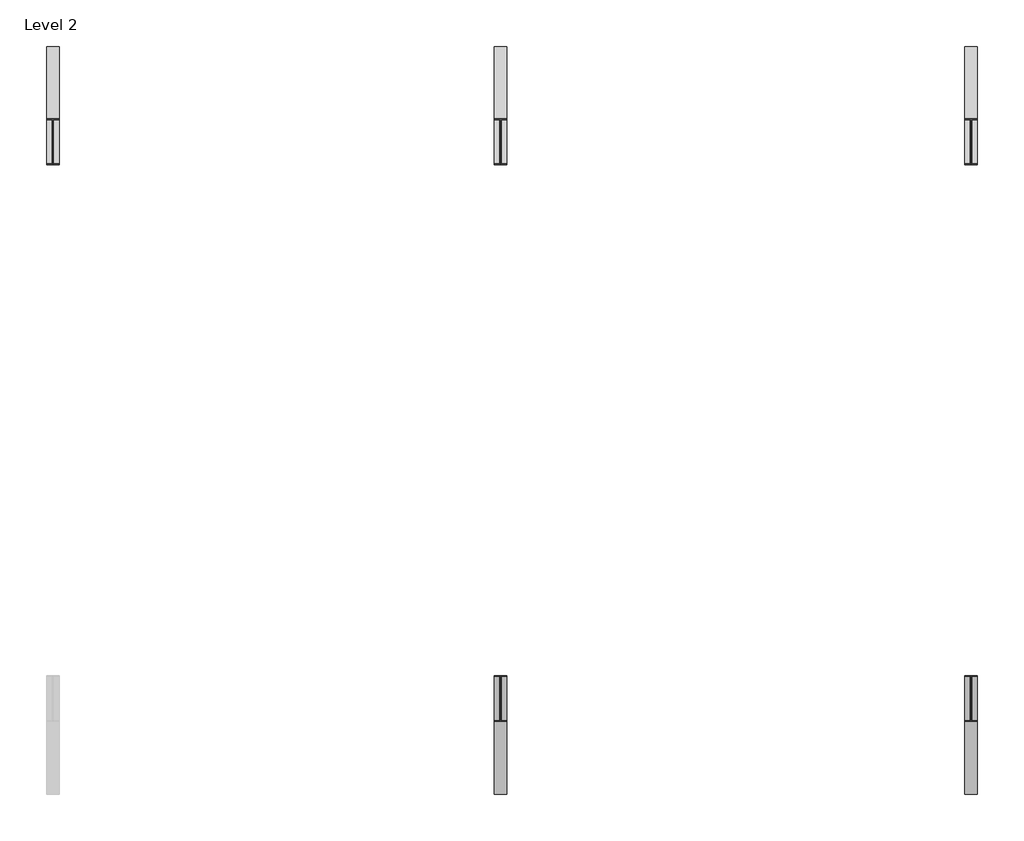
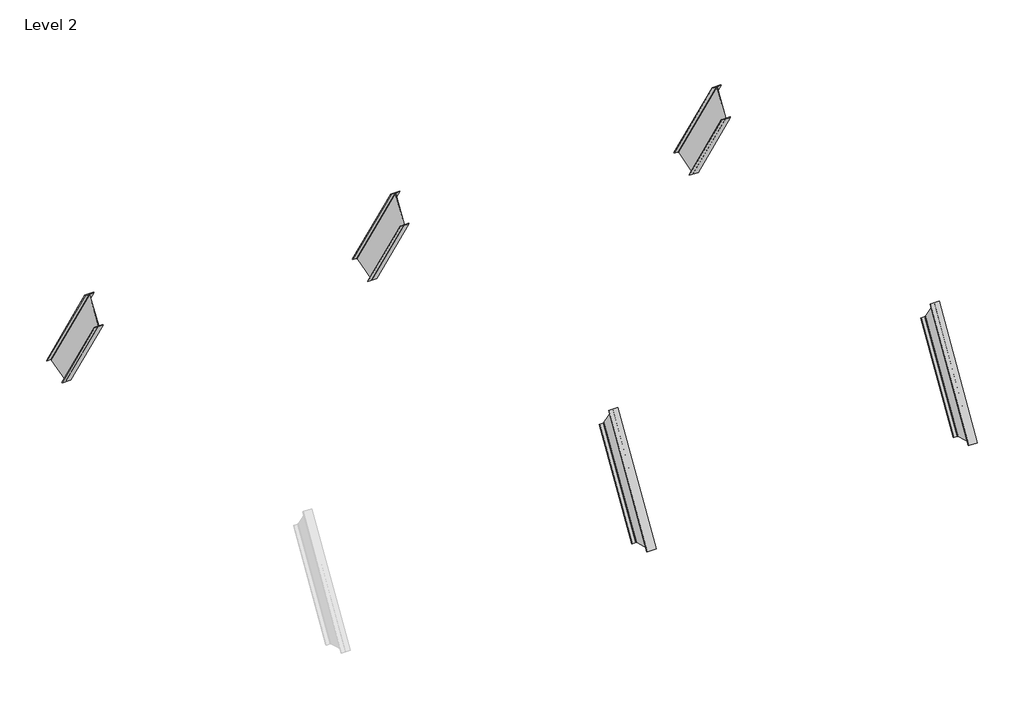
# One storey, part 2 of 2: 5 beams.
"""IFC4 building model written with IfcOpenShell, lengths in millimetres."""

from ifc_helpers import new_model, si_unit, frame, origin, place, context, project, spatial, polyline, ellipse_curve, element, save
from ifc_brep_helpers import plane_surface, revolved_surface, advanced_brep

model = new_model("IFC4")

# Units and contexts
model_context = context("Model", 3, world=origin())
ifc_project = project(units=[si_unit("LENGTHUNIT", "METRE", prefix="MILLI")], contexts=[model_context])

# Site, building, storey
site = spatial("IfcSite", under=ifc_project)
building = spatial("IfcBuilding", under=site)
storey = spatial("IfcBuildingStorey", under=building, Name="Level 2", Elevation=3048.0)

# Beams
placement = place(None, origin())
element("IfcBeam", 1, ObjectType="W Shapes : W 6X18.5", at=placement, inside=storey, context=model_context, shape_type="AdvancedBrep", body=[
    advanced_brep(
    [(28967.3280052, 10139.0601337, 4314.3781499), (29032.9870052, 10139.0601337, 4314.3781499), (29032.9870052, 11123.4136018, 2696.9143292), (28967.3280052, 11123.4136018, 2696.9143292), (28959.7080052, 10143.6843616, 4321.4371423), (28959.7080052, 11131.0336533, 2699.0506628), (28959.7080052, 10407.8819145, 4724.7409096), (28959.7080052, 11566.3925949, 2821.106522), (28967.3280052, 10412.5061424, 4731.799902), (28967.3280052, 11574.0126464, 2823.2428556), (29032.9870052, 10412.5061424, 4731.799902), (29032.9870052, 11574.0126464, 2823.2428556), (29032.9870052, 10418.3634977, 4740.7412924), (29032.9870052, 11583.6647116, 2825.9488782), (28880.5870052, 10418.3634977, 4740.7412924), (28880.5870052, 11583.6647116, 2825.9488782), (28880.5870052, 10412.5061424, 4731.799902), (28880.5870052, 11574.0126464, 2823.2428556), (28946.2460052, 10412.5061424, 4731.799902), (28946.2460052, 11574.0126464, 2823.2428556), (28953.8660052, 10407.8819145, 4724.7409096), (28953.8660052, 11566.3925949, 2821.106522), (28953.8660052, 10143.6843616, 4321.4371423), (28953.8660052, 11131.0336533, 2699.0506628), (28946.2460052, 10139.0601337, 4314.3781499), (28946.2460052, 11123.4136018, 2696.9143292), (28880.5870052, 10139.0601337, 4314.3781499), (28880.5870052, 11123.4136018, 2696.9143292), (28880.5870052, 10133.2027784, 4305.4367595), (28880.5870052, 11113.7615366, 2694.2083066), (29032.9870052, 10133.2027784, 4305.4367595), (29032.9870052, 11113.7615366, 2694.2083066)],
    [
        (0, 1),
        (1, 2),
        (2, 3),
        (3, 0),
        (4, 0, ellipse_curve(frame((28967.3280052, 10143.6843616, 4321.4371423), z_axis=(0.0, -0.836495308057375, 0.5479740866117643), x_axis=(0.0, -0.5479740866117645, -0.8364953080573748)), 8.4387711, 7.62)),
        (3, 5, ellipse_curve(frame((28967.3280052, 11131.0336533, 2699.0506628), z_axis=(0.0, 0.26994852802482067, -0.9628747541696338), x_axis=(0.0, 0.9628747541696336, 0.269948528024821)), 7.9138553, 7.62)),
        (5, 4),
        (6, 4),
        (5, 7),
        (7, 6),
        (8, 6, ellipse_curve(frame((28967.3280052, 10407.8819145, 4724.7409096), z_axis=(0.0, -0.836495308057375, 0.5479740866117643), x_axis=(0.0, -0.5479740866117645, -0.8364953080573748)), 8.4387711, 7.62)),
        (7, 9, ellipse_curve(frame((28967.3280052, 11566.3925949, 2821.106522), z_axis=(0.0, 0.26994852802482067, -0.9628747541696338), x_axis=(0.0, 0.9628747541696336, 0.269948528024821)), 7.9138553, 7.62)),
        (9, 8),
        (10, 8),
        (9, 11),
        (11, 10),
        (12, 10),
        (11, 13),
        (13, 12),
        (14, 12),
        (13, 15),
        (15, 14),
        (16, 14),
        (15, 17),
        (17, 16),
        (18, 16),
        (17, 19),
        (19, 18),
        (20, 18, ellipse_curve(frame((28946.2460052, 10407.8819145, 4724.7409096), z_axis=(0.0, -0.836495308057375, 0.5479740866117643), x_axis=(0.0, -0.5479740866117645, -0.8364953080573748)), 8.4387711, 7.62)),
        (19, 21, ellipse_curve(frame((28946.2460052, 11566.3925949, 2821.106522), z_axis=(0.0, 0.26994852802482067, -0.9628747541696338), x_axis=(0.0, 0.9628747541696336, 0.269948528024821)), 7.9138553, 7.62)),
        (21, 20),
        (22, 20),
        (21, 23),
        (23, 22),
        (24, 22, ellipse_curve(frame((28946.2460052, 10143.6843616, 4321.4371423), z_axis=(0.0, -0.836495308057375, 0.5479740866117643), x_axis=(0.0, -0.5479740866117645, -0.8364953080573748)), 8.4387711, 7.62)),
        (23, 25, ellipse_curve(frame((28946.2460052, 11131.0336533, 2699.0506628), z_axis=(0.0, 0.26994852802482067, -0.9628747541696338), x_axis=(0.0, 0.9628747541696336, 0.269948528024821)), 7.9138553, 7.62)),
        (25, 24),
        (26, 24),
        (25, 27),
        (27, 26),
        (28, 26),
        (27, 29),
        (29, 28),
        (30, 28),
        (29, 31),
        (31, 30),
        (1, 30),
        (31, 2),
    ],
    [
        plane_surface(frame((29032.9870052, 10025.1990543, 4501.4716915), z_axis=(0.0, 0.8542430559708922, 0.5198738321222864), x_axis=(0.0, 0.5198738321222864, -0.8542430559708922))),
        revolved_surface(polyline([(28959.708005200002, 11132.144372669503, 2697.225557775976), (28959.708005200002, 10141.799257339859, 4324.534696094065)]), (28967.3280052, 10031.7083863, 4505.4331301), (0.0, 0.5198738321222863, -0.8542430559708921)),
        plane_surface(frame((28959.7080052, 10031.7083863, 4505.4331301), z_axis=(1.0000000000000002, 0.0, 0.0), x_axis=(0.0, 0.5198738321222864, -0.8542430559708922))),
        revolved_surface(polyline([(28959.708005200002, 11567.50331433201, 2819.281417010493), (28959.708005200002, 10405.996810289686, 4727.8384634243885)]), (28967.3280052, 10403.6082262, 4731.7633222), (0.0, 0.5198738321222863, -0.8542430559708921)),
        plane_surface(frame((28967.3280052, 10410.1175583, 4735.7247608), z_axis=(0.0, -0.8542430559708922, -0.5198738321222864), x_axis=(0.0, 0.5198738321222864, -0.8542430559708922))),
        plane_surface(frame((29032.9870052, 10410.1175583, 4735.7247608), z_axis=(1.0000000000000002, 0.0, 0.0), x_axis=(0.0, 0.5198738321222864, -0.8542430559708922))),
        plane_surface(frame((29032.9870052, 10418.3627123, 4740.742583), z_axis=(0.0, 0.8542430559708922, 0.5198738321222864), x_axis=(0.0, 0.5198738321222864, -0.8542430559708922))),
        plane_surface(frame((28880.5870052, 10418.3627123, 4740.742583), z_axis=(-1.0000000000000002, 0.0, 0.0), x_axis=(0.0, 0.5198738321222864, -0.8542430559708922))),
        plane_surface(frame((28880.5870052, 10410.1175583, 4735.7247608), z_axis=(0.0, -0.8542430559708922, -0.5198738321222864), x_axis=(0.0, 0.5198738321222864, -0.8542430559708922))),
        revolved_surface(polyline([(28938.6260052, 11567.50331433201, 2819.281417010493), (28938.6260052, 10405.996810289686, 4727.8384634243885)]), (28946.2460052, 10403.6082262, 4731.7633222), (0.0, 0.5198738321222863, -0.8542430559708921)),
        plane_surface(frame((28953.8660052, 10403.6082262, 4731.7633222), z_axis=(-1.0000000000000002, 0.0, 0.0), x_axis=(0.0, 0.5198738321222864, -0.8542430559708922))),
        revolved_surface(polyline([(28938.6260052, 11132.144372669503, 2697.225557775976), (28938.6260052, 10141.799257339859, 4324.534696094065)]), (28946.2460052, 10031.7083863, 4505.4331301), (0.0, 0.5198738321222863, -0.8542430559708921)),
        plane_surface(frame((28946.2460052, 10025.1990543, 4501.4716915), z_axis=(0.0, 0.8542430559708922, 0.5198738321222864), x_axis=(0.0, 0.5198738321222864, -0.8542430559708922))),
        plane_surface(frame((28880.5870052, 10025.1990543, 4501.4716915), z_axis=(-1.0000000000000002, 0.0, 0.0), x_axis=(0.0, 0.5198738321222864, -0.8542430559708922))),
        plane_surface(frame((28880.5870052, 10016.9539003, 4496.4538693), z_axis=(0.0, -0.8542430559708922, -0.5198738321222864), x_axis=(0.0, 0.5198738321222864, -0.8542430559708922))),
        plane_surface(frame((29032.9870052, 10016.9539003, 4496.4538693), z_axis=(1.0000000000000002, 0.0, 0.0), x_axis=(0.0, 0.5198738321222864, -0.8542430559708922))),
        plane_surface(frame((28956.7905771, 10418.3654245, 4740.7442336), z_axis=(0.0, -0.836495308057375, 0.5479740866117643), x_axis=(1.0, 0.0, 0.0))),
        plane_surface(frame((31332.3254456, 11714.3703228, 2862.5930909), z_axis=(0.0, 0.26994852802482067, -0.9628747541696338), x_axis=(-1.0, 0.0, 0.0))),
    ],
    [
        (0, [[1, 2, 3, 4]]),
        (1, [[5, -4, 6, 7]]),
        (2, [[8, -7, 9, 10]]),
        (3, [[11, -10, 12, 13]]),
        (4, [[14, -13, 15, 16]]),
        (5, [[17, -16, 18, 19]]),
        (6, [[20, -19, 21, 22]]),
        (7, [[23, -22, 24, 25]]),
        (8, [[26, -25, 27, 28]]),
        (9, [[29, -28, 30, 31]]),
        (10, [[32, -31, 33, 34]]),
        (11, [[35, -34, 36, 37]]),
        (12, [[38, -37, 39, 40]]),
        (13, [[41, -40, 42, 43]]),
        (14, [[44, -43, 45, 46]]),
        (15, [[47, -46, 48, -2]]),
        (16, [[-1, -5, -8, -11, -14, -17, -20, -23, -26, -29, -32, -35, -38, -41, -44, -47]]),
        (17, [[-3, -48, -45, -42, -39, -36, -33, -30, -27, -24, -21, -18, -15, -12, -9, -6]]),
    ],
),
])
element("IfcBeam", 2, ObjectType="W Shapes : W 6X18.5", at=placement, inside=storey, context=model_context, shape_type="AdvancedBrep", body=[
    advanced_brep(
    [(29032.9870052, 4087.4629396, 4314.3781499), (28967.3280052, 4087.4629396, 4314.3781499), (28967.3280052, 3103.1094714, 2696.9143292), (29032.9870052, 3103.1094714, 2696.9143292), (28959.7080052, 4082.8387117, 4321.4371423), (28959.7080052, 3095.4894199, 2699.0506628), (28959.7080052, 3818.6411587, 4724.7409096), (28959.7080052, 2660.1304783, 2821.106522), (28967.3280052, 3814.0169308, 4731.799902), (28967.3280052, 2652.5104268, 2823.2428556), (29032.9870052, 3814.0169308, 4731.799902), (29032.9870052, 2652.5104268, 2823.2428556), (29032.9870052, 3808.1595755, 4740.7412924), (29032.9870052, 2642.8583616, 2825.9488782), (28880.5870052, 3808.1595755, 4740.7412924), (28880.5870052, 2642.8583616, 2825.9488782), (28880.5870052, 3814.0169308, 4731.799902), (28880.5870052, 2652.5104268, 2823.2428556), (28946.2460052, 3814.0169308, 4731.799902), (28946.2460052, 2652.5104268, 2823.2428556), (28953.8660052, 3818.6411587, 4724.7409096), (28953.8660052, 2660.1304783, 2821.106522), (28953.8660052, 4082.8387117, 4321.4371423), (28953.8660052, 3095.4894199, 2699.0506628), (28946.2460052, 4087.4629396, 4314.3781499), (28946.2460052, 3103.1094714, 2696.9143292), (28880.5870052, 4087.4629396, 4314.3781499), (28880.5870052, 3103.1094714, 2696.9143292), (28880.5870052, 4093.3202949, 4305.4367595), (28880.5870052, 3112.7615366, 2694.2083066), (29032.9870052, 4093.3202949, 4305.4367595), (29032.9870052, 3112.7615366, 2694.2083066)],
    [
        (0, 1),
        (1, 2),
        (2, 3),
        (3, 0),
        (1, 4, ellipse_curve(frame((28967.3280052, 4082.8387117, 4321.4371423), z_axis=(0.0, 0.8364953080573764, 0.5479740866117624), x_axis=(0.0, 0.5479740866117631, -0.8364953080573758)), 8.4387711, 7.62)),
        (4, 5),
        (5, 2, ellipse_curve(frame((28967.3280052, 3095.4894199, 2699.0506628), z_axis=(0.0, -0.26994852802482067, -0.9628747541696338), x_axis=(0.0, -0.9628747541696336, 0.26994852802482094)), 7.9138553, 7.62)),
        (4, 6),
        (6, 7),
        (7, 5),
        (6, 8, ellipse_curve(frame((28967.3280052, 3818.6411587, 4724.7409096), z_axis=(0.0, 0.8364953080573764, 0.5479740866117624), x_axis=(0.0, 0.5479740866117631, -0.8364953080573758)), 8.4387711, 7.62)),
        (8, 9),
        (9, 7, ellipse_curve(frame((28967.3280052, 2660.1304783, 2821.106522), z_axis=(0.0, -0.26994852802482067, -0.9628747541696338), x_axis=(0.0, -0.9628747541696336, 0.26994852802482094)), 7.9138553, 7.62)),
        (8, 10),
        (10, 11),
        (11, 9),
        (10, 12),
        (12, 13),
        (13, 11),
        (12, 14),
        (14, 15),
        (15, 13),
        (14, 16),
        (16, 17),
        (17, 15),
        (16, 18),
        (18, 19),
        (19, 17),
        (18, 20, ellipse_curve(frame((28946.2460052, 3818.6411587, 4724.7409096), z_axis=(0.0, 0.8364953080573764, 0.5479740866117624), x_axis=(0.0, 0.5479740866117631, -0.8364953080573758)), 8.4387711, 7.62)),
        (20, 21),
        (21, 19, ellipse_curve(frame((28946.2460052, 2660.1304783, 2821.106522), z_axis=(0.0, -0.26994852802482067, -0.9628747541696338), x_axis=(0.0, -0.9628747541696336, 0.26994852802482094)), 7.9138553, 7.62)),
        (20, 22),
        (22, 23),
        (23, 21),
        (22, 24, ellipse_curve(frame((28946.2460052, 4082.8387117, 4321.4371423), z_axis=(0.0, 0.8364953080573764, 0.5479740866117624), x_axis=(0.0, 0.5479740866117631, -0.8364953080573758)), 8.4387711, 7.62)),
        (24, 25),
        (25, 23, ellipse_curve(frame((28946.2460052, 3095.4894199, 2699.0506628), z_axis=(0.0, -0.26994852802482067, -0.9628747541696338), x_axis=(0.0, -0.9628747541696336, 0.26994852802482094)), 7.9138553, 7.62)),
        (24, 26),
        (26, 27),
        (27, 25),
        (26, 28),
        (28, 29),
        (29, 27),
        (28, 30),
        (30, 31),
        (31, 29),
        (30, 0),
        (3, 31),
    ],
    [
        plane_surface(frame((29032.9870052, 4201.324019, 4501.4716915), z_axis=(0.0, -0.8542430559708922, 0.5198738321222864), x_axis=(0.0, -0.5198738321222864, -0.8542430559708922))),
        revolved_surface(polyline([(28959.708005200002, 3094.3787005304976, 2697.225557775975), (28959.708005200002, 4084.7238158871687, 4324.534696138475)]), (28967.3280052, 4194.8146869, 4505.4331301), (0.0, -0.5198738321222864, -0.8542430559708922)),
        plane_surface(frame((28959.7080052, 4194.8146869, 4505.4331301), z_axis=(1.0000000000000002, 0.0, 0.0), x_axis=(0.0, -0.5198738321222864, -0.8542430559708922))),
        revolved_surface(polyline([(28959.708005200002, 2659.0197588679885, 2819.2814170104925), (28959.708005200002, 3820.5262629103145, 4727.8384634243885)]), (28967.3280052, 3822.914847, 4731.7633222), (0.0, -0.5198738321222864, -0.8542430559708922)),
        plane_surface(frame((28967.3280052, 3816.405515, 4735.7247608), z_axis=(0.0, 0.8542430559708922, -0.5198738321222864), x_axis=(0.0, -0.5198738321222864, -0.8542430559708922))),
        plane_surface(frame((29032.9870052, 3816.405515, 4735.7247608), z_axis=(1.0000000000000002, 0.0, 0.0), x_axis=(0.0, -0.5198738321222864, -0.8542430559708922))),
        plane_surface(frame((29032.9870052, 3808.160361, 4740.742583), z_axis=(0.0, -0.8542430559708922, 0.5198738321222864), x_axis=(0.0, -0.5198738321222864, -0.8542430559708922))),
        plane_surface(frame((28880.5870052, 3808.160361, 4740.742583), z_axis=(-1.0000000000000002, 0.0, 0.0), x_axis=(0.0, -0.5198738321222864, -0.8542430559708922))),
        plane_surface(frame((28880.5870052, 3816.405515, 4735.7247608), z_axis=(0.0, 0.8542430559708922, -0.5198738321222864), x_axis=(0.0, -0.5198738321222864, -0.8542430559708922))),
        revolved_surface(polyline([(28938.6260052, 2659.0197588679885, 2819.2814170104925), (28938.6260052, 3820.5262629103145, 4727.8384634243885)]), (28946.2460052, 3822.914847, 4731.7633222), (0.0, -0.5198738321222864, -0.8542430559708922)),
        plane_surface(frame((28953.8660052, 3822.914847, 4731.7633222), z_axis=(-1.0000000000000002, 0.0, 0.0), x_axis=(0.0, -0.5198738321222864, -0.8542430559708922))),
        revolved_surface(polyline([(28938.6260052, 3094.3787005304976, 2697.225557775975), (28938.6260052, 4084.7238158871687, 4324.534696138475)]), (28946.2460052, 4194.8146869, 4505.4331301), (0.0, -0.5198738321222864, -0.8542430559708922)),
        plane_surface(frame((28946.2460052, 4201.324019, 4501.4716915), z_axis=(0.0, -0.8542430559708922, 0.5198738321222864), x_axis=(0.0, -0.5198738321222864, -0.8542430559708922))),
        plane_surface(frame((28880.5870052, 4201.324019, 4501.4716915), z_axis=(-1.0000000000000002, 0.0, 0.0), x_axis=(0.0, -0.5198738321222864, -0.8542430559708922))),
        plane_surface(frame((28880.5870052, 4209.569173, 4496.4538693), z_axis=(0.0, 0.8542430559708922, -0.5198738321222864), x_axis=(0.0, -0.5198738321222864, -0.8542430559708922))),
        plane_surface(frame((29032.9870052, 4209.569173, 4496.4538693), z_axis=(1.0000000000000002, 0.0, 0.0), x_axis=(0.0, -0.5198738321222864, -0.8542430559708922))),
        plane_surface(frame((26581.2485648, 2512.1527504, 2862.5930909), z_axis=(0.0, -0.26994852802482067, -0.9628747541696338), x_axis=(1.0, 0.0, 0.0))),
        plane_surface(frame((28956.7905771, 4093.3183681, 4305.4397008), z_axis=(0.0, 0.8364953080573764, 0.5479740866117624), x_axis=(1.0, 0.0, 0.0))),
    ],
    [
        (0, [[1, 2, 3, 4]]),
        (1, [[5, 6, 7, -2]]),
        (2, [[8, 9, 10, -6]]),
        (3, [[11, 12, 13, -9]]),
        (4, [[14, 15, 16, -12]]),
        (5, [[17, 18, 19, -15]]),
        (6, [[20, 21, 22, -18]]),
        (7, [[23, 24, 25, -21]]),
        (8, [[26, 27, 28, -24]]),
        (9, [[29, 30, 31, -27]]),
        (10, [[32, 33, 34, -30]]),
        (11, [[35, 36, 37, -33]]),
        (12, [[38, 39, 40, -36]]),
        (13, [[41, 42, 43, -39]]),
        (14, [[44, 45, 46, -42]]),
        (15, [[47, -4, 48, -45]]),
        (16, [[-3, -7, -10, -13, -16, -19, -22, -25, -28, -31, -34, -37, -40, -43, -46, -48]]),
        (17, [[-1, -47, -44, -41, -38, -35, -32, -29, -26, -23, -20, -17, -14, -11, -8, -5]]),
    ],
),
])
element("IfcBeam", 3, ObjectType="W Shapes : W 6X18.5", at=placement, inside=storey, context=model_context, shape_type="AdvancedBrep", body=[
    advanced_brep(
    [(23341.2280052, 10139.0601337, 4314.3781499), (23406.8870052, 10139.0601337, 4314.3781499), (23406.8870052, 11123.4136018, 2696.9143292), (23341.2280052, 11123.4136018, 2696.9143292), (23333.6080052, 10143.6843616, 4321.4371423), (23333.6080052, 11131.0336533, 2699.0506628), (23333.6080052, 10407.8819145, 4724.7409096), (23333.6080052, 11566.3925949, 2821.106522), (23341.2280052, 10412.5061424, 4731.799902), (23341.2280052, 11574.0126464, 2823.2428556), (23406.8870052, 10412.5061424, 4731.799902), (23406.8870052, 11574.0126464, 2823.2428556), (23406.8870052, 10418.3634977, 4740.7412924), (23406.8870052, 11583.6647116, 2825.9488782), (23254.4870052, 10418.3634977, 4740.7412924), (23254.4870052, 11583.6647116, 2825.9488782), (23254.4870052, 10412.5061424, 4731.799902), (23254.4870052, 11574.0126464, 2823.2428556), (23320.1460052, 10412.5061424, 4731.799902), (23320.1460052, 11574.0126464, 2823.2428556), (23327.7660052, 10407.8819145, 4724.7409096), (23327.7660052, 11566.3925949, 2821.106522), (23327.7660052, 10143.6843616, 4321.4371423), (23327.7660052, 11131.0336533, 2699.0506628), (23320.1460052, 10139.0601337, 4314.3781499), (23320.1460052, 11123.4136018, 2696.9143292), (23254.4870052, 10139.0601337, 4314.3781499), (23254.4870052, 11123.4136018, 2696.9143292), (23254.4870052, 10133.2027784, 4305.4367595), (23254.4870052, 11113.7615366, 2694.2083066), (23406.8870052, 10133.2027784, 4305.4367595), (23406.8870052, 11113.7615366, 2694.2083066)],
    [
        (0, 1),
        (1, 2),
        (2, 3),
        (3, 0),
        (4, 0, ellipse_curve(frame((23341.2280052, 10143.6843616, 4321.4371423), z_axis=(0.0, -0.836495308057375, 0.5479740866117643), x_axis=(0.0, -0.5479740866117645, -0.8364953080573748)), 8.4387711, 7.62)),
        (3, 5, ellipse_curve(frame((23341.2280052, 11131.0336533, 2699.0506628), z_axis=(0.0, 0.2699485280248213, -0.9628747541696336), x_axis=(0.0, 0.9628747541696333, 0.26994852802482194)), 7.9138553, 7.62)),
        (5, 4),
        (6, 4),
        (5, 7),
        (7, 6),
        (8, 6, ellipse_curve(frame((23341.2280052, 10407.8819145, 4724.7409096), z_axis=(0.0, -0.836495308057375, 0.5479740866117643), x_axis=(0.0, -0.5479740866117645, -0.8364953080573748)), 8.4387711, 7.62)),
        (7, 9, ellipse_curve(frame((23341.2280052, 11566.3925949, 2821.106522), z_axis=(0.0, 0.2699485280248213, -0.9628747541696336), x_axis=(0.0, 0.9628747541696333, 0.26994852802482194)), 7.9138553, 7.62)),
        (9, 8),
        (10, 8),
        (9, 11),
        (11, 10),
        (12, 10),
        (11, 13),
        (13, 12),
        (14, 12),
        (13, 15),
        (15, 14),
        (16, 14),
        (15, 17),
        (17, 16),
        (18, 16),
        (17, 19),
        (19, 18),
        (20, 18, ellipse_curve(frame((23320.1460052, 10407.8819145, 4724.7409096), z_axis=(0.0, -0.836495308057375, 0.5479740866117643), x_axis=(0.0, -0.5479740866117645, -0.8364953080573748)), 8.4387711, 7.62)),
        (19, 21, ellipse_curve(frame((23320.1460052, 11566.3925949, 2821.106522), z_axis=(0.0, 0.2699485280248213, -0.9628747541696336), x_axis=(0.0, 0.9628747541696333, 0.26994852802482194)), 7.9138553, 7.62)),
        (21, 20),
        (22, 20),
        (21, 23),
        (23, 22),
        (24, 22, ellipse_curve(frame((23320.1460052, 10143.6843616, 4321.4371423), z_axis=(0.0, -0.836495308057375, 0.5479740866117643), x_axis=(0.0, -0.5479740866117645, -0.8364953080573748)), 8.4387711, 7.62)),
        (23, 25, ellipse_curve(frame((23320.1460052, 11131.0336533, 2699.0506628), z_axis=(0.0, 0.2699485280248213, -0.9628747541696336), x_axis=(0.0, 0.9628747541696333, 0.26994852802482194)), 7.9138553, 7.62)),
        (25, 24),
        (26, 24),
        (25, 27),
        (27, 26),
        (28, 26),
        (27, 29),
        (29, 28),
        (30, 28),
        (29, 31),
        (31, 30),
        (1, 30),
        (31, 2),
    ],
    [
        plane_surface(frame((23406.8870052, 10025.1990543, 4501.4716915), z_axis=(0.0, 0.8542430559708922, 0.5198738321222864), x_axis=(0.0, 0.5198738321222864, -0.8542430559708922))),
        revolved_surface(polyline([(23333.6080052, 11132.144372669503, 2697.225557775976), (23333.6080052, 10141.799257339859, 4324.534696094065)]), (23341.2280052, 10031.7083863, 4505.4331301), (0.0, 0.5198738321222863, -0.8542430559708921)),
        plane_surface(frame((23333.6080052, 10031.7083863, 4505.4331301), z_axis=(1.0000000000000002, 0.0, 0.0), x_axis=(0.0, 0.5198738321222864, -0.8542430559708922))),
        revolved_surface(polyline([(23333.6080052, 11567.50331433201, 2819.281417010493), (23333.6080052, 10405.996810289686, 4727.8384634243885)]), (23341.2280052, 10403.6082262, 4731.7633222), (0.0, 0.5198738321222863, -0.8542430559708921)),
        plane_surface(frame((23341.2280052, 10410.1175583, 4735.7247608), z_axis=(0.0, -0.8542430559708922, -0.5198738321222864), x_axis=(0.0, 0.5198738321222864, -0.8542430559708922))),
        plane_surface(frame((23406.8870052, 10410.1175583, 4735.7247608), z_axis=(1.0000000000000002, 0.0, 0.0), x_axis=(0.0, 0.5198738321222864, -0.8542430559708922))),
        plane_surface(frame((23406.8870052, 10418.3627123, 4740.742583), z_axis=(0.0, 0.8542430559708922, 0.5198738321222864), x_axis=(0.0, 0.5198738321222864, -0.8542430559708922))),
        plane_surface(frame((23254.4870052, 10418.3627123, 4740.742583), z_axis=(-1.0000000000000002, 0.0, 0.0), x_axis=(0.0, 0.5198738321222864, -0.8542430559708922))),
        plane_surface(frame((23254.4870052, 10410.1175583, 4735.7247608), z_axis=(0.0, -0.8542430559708922, -0.5198738321222864), x_axis=(0.0, 0.5198738321222864, -0.8542430559708922))),
        revolved_surface(polyline([(23312.5260052, 11567.50331433201, 2819.281417010493), (23312.5260052, 10405.996810289686, 4727.8384634243885)]), (23320.1460052, 10403.6082262, 4731.7633222), (0.0, 0.5198738321222863, -0.8542430559708921)),
        plane_surface(frame((23327.7660052, 10403.6082262, 4731.7633222), z_axis=(-1.0000000000000002, 0.0, 0.0), x_axis=(0.0, 0.5198738321222864, -0.8542430559708922))),
        revolved_surface(polyline([(23312.5260052, 11132.144372669503, 2697.225557775976), (23312.5260052, 10141.799257339859, 4324.534696094065)]), (23320.1460052, 10031.7083863, 4505.4331301), (0.0, 0.5198738321222863, -0.8542430559708921)),
        plane_surface(frame((23320.1460052, 10025.1990543, 4501.4716915), z_axis=(0.0, 0.8542430559708922, 0.5198738321222864), x_axis=(0.0, 0.5198738321222864, -0.8542430559708922))),
        plane_surface(frame((23254.4870052, 10025.1990543, 4501.4716915), z_axis=(-1.0000000000000002, 0.0, 0.0), x_axis=(0.0, 0.5198738321222864, -0.8542430559708922))),
        plane_surface(frame((23254.4870052, 10016.9539003, 4496.4538693), z_axis=(0.0, -0.8542430559708922, -0.5198738321222864), x_axis=(0.0, 0.5198738321222864, -0.8542430559708922))),
        plane_surface(frame((23406.8870052, 10016.9539003, 4496.4538693), z_axis=(1.0000000000000002, 0.0, 0.0), x_axis=(0.0, 0.5198738321222864, -0.8542430559708922))),
        plane_surface(frame((25706.2254456, 11714.3703228, 2862.5930909), z_axis=(0.0, 0.2699485280248213, -0.9628747541696336), x_axis=(-1.0, 0.0, 0.0))),
        plane_surface(frame((23330.6905771, 10418.3654245, 4740.7442336), z_axis=(0.0, -0.836495308057375, 0.5479740866117643), x_axis=(1.0, 0.0, 0.0))),
    ],
    [
        (0, [[1, 2, 3, 4]]),
        (1, [[5, -4, 6, 7]]),
        (2, [[8, -7, 9, 10]]),
        (3, [[11, -10, 12, 13]]),
        (4, [[14, -13, 15, 16]]),
        (5, [[17, -16, 18, 19]]),
        (6, [[20, -19, 21, 22]]),
        (7, [[23, -22, 24, 25]]),
        (8, [[26, -25, 27, 28]]),
        (9, [[29, -28, 30, 31]]),
        (10, [[32, -31, 33, 34]]),
        (11, [[35, -34, 36, 37]]),
        (12, [[38, -37, 39, 40]]),
        (13, [[41, -40, 42, 43]]),
        (14, [[44, -43, 45, 46]]),
        (15, [[47, -46, 48, -2]]),
        (16, [[-3, -48, -45, -42, -39, -36, -33, -30, -27, -24, -21, -18, -15, -12, -9, -6]]),
        (17, [[-1, -5, -8, -11, -14, -17, -20, -23, -26, -29, -32, -35, -38, -41, -44, -47]]),
    ],
),
])
element("IfcBeam", 4, ObjectType="W Shapes : W 6X18.5", at=placement, inside=storey, context=model_context, shape_type="AdvancedBrep", body=[
    advanced_brep(
    [(23406.8870052, 4087.4629396, 4314.3781499), (23341.2280052, 4087.4629396, 4314.3781499), (23341.2280052, 3103.1094714, 2696.9143292), (23406.8870052, 3103.1094714, 2696.9143292), (23333.6080052, 4082.8387117, 4321.4371423), (23333.6080052, 3095.4894199, 2699.0506628), (23333.6080052, 3818.6411587, 4724.7409096), (23333.6080052, 2660.1304783, 2821.106522), (23341.2280052, 3814.0169308, 4731.799902), (23341.2280052, 2652.5104268, 2823.2428556), (23406.8870052, 3814.0169308, 4731.799902), (23406.8870052, 2652.5104268, 2823.2428556), (23406.8870052, 3808.1595755, 4740.7412924), (23406.8870052, 2642.8583616, 2825.9488782), (23254.4870052, 3808.1595755, 4740.7412924), (23254.4870052, 2642.8583616, 2825.9488782), (23254.4870052, 3814.0169308, 4731.799902), (23254.4870052, 2652.5104268, 2823.2428556), (23320.1460052, 3814.0169308, 4731.799902), (23320.1460052, 2652.5104268, 2823.2428556), (23327.7660052, 3818.6411587, 4724.7409096), (23327.7660052, 2660.1304783, 2821.106522), (23327.7660052, 4082.8387117, 4321.4371423), (23327.7660052, 3095.4894199, 2699.0506628), (23320.1460052, 4087.4629396, 4314.3781499), (23320.1460052, 3103.1094714, 2696.9143292), (23254.4870052, 4087.4629396, 4314.3781499), (23254.4870052, 3103.1094714, 2696.9143292), (23254.4870052, 4093.3202949, 4305.4367595), (23254.4870052, 3112.7615366, 2694.2083066), (23406.8870052, 4093.3202949, 4305.4367595), (23406.8870052, 3112.7615366, 2694.2083066)],
    [
        (0, 1),
        (1, 2),
        (2, 3),
        (3, 0),
        (1, 4, ellipse_curve(frame((23341.2280052, 4082.8387117, 4321.4371423), z_axis=(0.0, 0.8364953080573764, 0.5479740866117624), x_axis=(0.0, 0.5479740866117631, -0.8364953080573758)), 8.4387711, 7.62)),
        (4, 5),
        (5, 2, ellipse_curve(frame((23341.2280052, 3095.4894199, 2699.0506628), z_axis=(0.0, -0.26994852802482067, -0.9628747541696338), x_axis=(0.0, -0.9628747541696336, 0.26994852802482094)), 7.9138553, 7.62)),
        (4, 6),
        (6, 7),
        (7, 5),
        (6, 8, ellipse_curve(frame((23341.2280052, 3818.6411587, 4724.7409096), z_axis=(0.0, 0.8364953080573764, 0.5479740866117624), x_axis=(0.0, 0.5479740866117631, -0.8364953080573758)), 8.4387711, 7.62)),
        (8, 9),
        (9, 7, ellipse_curve(frame((23341.2280052, 2660.1304783, 2821.106522), z_axis=(0.0, -0.26994852802482067, -0.9628747541696338), x_axis=(0.0, -0.9628747541696336, 0.26994852802482094)), 7.9138553, 7.62)),
        (8, 10),
        (10, 11),
        (11, 9),
        (10, 12),
        (12, 13),
        (13, 11),
        (12, 14),
        (14, 15),
        (15, 13),
        (14, 16),
        (16, 17),
        (17, 15),
        (16, 18),
        (18, 19),
        (19, 17),
        (18, 20, ellipse_curve(frame((23320.1460052, 3818.6411587, 4724.7409096), z_axis=(0.0, 0.8364953080573764, 0.5479740866117624), x_axis=(0.0, 0.5479740866117631, -0.8364953080573758)), 8.4387711, 7.62)),
        (20, 21),
        (21, 19, ellipse_curve(frame((23320.1460052, 2660.1304783, 2821.106522), z_axis=(0.0, -0.26994852802482067, -0.9628747541696338), x_axis=(0.0, -0.9628747541696336, 0.26994852802482094)), 7.9138553, 7.62)),
        (20, 22),
        (22, 23),
        (23, 21),
        (22, 24, ellipse_curve(frame((23320.1460052, 4082.8387117, 4321.4371423), z_axis=(0.0, 0.8364953080573764, 0.5479740866117624), x_axis=(0.0, 0.5479740866117631, -0.8364953080573758)), 8.4387711, 7.62)),
        (24, 25),
        (25, 23, ellipse_curve(frame((23320.1460052, 3095.4894199, 2699.0506628), z_axis=(0.0, -0.26994852802482067, -0.9628747541696338), x_axis=(0.0, -0.9628747541696336, 0.26994852802482094)), 7.9138553, 7.62)),
        (24, 26),
        (26, 27),
        (27, 25),
        (26, 28),
        (28, 29),
        (29, 27),
        (28, 30),
        (30, 31),
        (31, 29),
        (30, 0),
        (3, 31),
    ],
    [
        plane_surface(frame((23406.8870052, 4201.324019, 4501.4716915), z_axis=(0.0, -0.8542430559708922, 0.5198738321222864), x_axis=(0.0, -0.5198738321222864, -0.8542430559708922))),
        revolved_surface(polyline([(23333.6080052, 3094.3787005304976, 2697.225557775975), (23333.6080052, 4084.7238158871687, 4324.534696138475)]), (23341.2280052, 4194.8146869, 4505.4331301), (0.0, -0.5198738321222864, -0.8542430559708922)),
        plane_surface(frame((23333.6080052, 4194.8146869, 4505.4331301), z_axis=(1.0000000000000002, 0.0, 0.0), x_axis=(0.0, -0.5198738321222864, -0.8542430559708922))),
        revolved_surface(polyline([(23333.6080052, 2659.0197588679885, 2819.2814170104925), (23333.6080052, 3820.5262629103145, 4727.8384634243885)]), (23341.2280052, 3822.914847, 4731.7633222), (0.0, -0.5198738321222864, -0.8542430559708922)),
        plane_surface(frame((23341.2280052, 3816.405515, 4735.7247608), z_axis=(0.0, 0.8542430559708922, -0.5198738321222864), x_axis=(0.0, -0.5198738321222864, -0.8542430559708922))),
        plane_surface(frame((23406.8870052, 3816.405515, 4735.7247608), z_axis=(1.0000000000000002, 0.0, 0.0), x_axis=(0.0, -0.5198738321222864, -0.8542430559708922))),
        plane_surface(frame((23406.8870052, 3808.160361, 4740.742583), z_axis=(0.0, -0.8542430559708922, 0.5198738321222864), x_axis=(0.0, -0.5198738321222864, -0.8542430559708922))),
        plane_surface(frame((23254.4870052, 3808.160361, 4740.742583), z_axis=(-1.0000000000000002, 0.0, 0.0), x_axis=(0.0, -0.5198738321222864, -0.8542430559708922))),
        plane_surface(frame((23254.4870052, 3816.405515, 4735.7247608), z_axis=(0.0, 0.8542430559708922, -0.5198738321222864), x_axis=(0.0, -0.5198738321222864, -0.8542430559708922))),
        revolved_surface(polyline([(23312.5260052, 2659.0197588679885, 2819.2814170104925), (23312.5260052, 3820.5262629103145, 4727.8384634243885)]), (23320.1460052, 3822.914847, 4731.7633222), (0.0, -0.5198738321222864, -0.8542430559708922)),
        plane_surface(frame((23327.7660052, 3822.914847, 4731.7633222), z_axis=(-1.0000000000000002, 0.0, 0.0), x_axis=(0.0, -0.5198738321222864, -0.8542430559708922))),
        revolved_surface(polyline([(23312.5260052, 3094.3787005304976, 2697.225557775975), (23312.5260052, 4084.7238158871687, 4324.534696138475)]), (23320.1460052, 4194.8146869, 4505.4331301), (0.0, -0.5198738321222864, -0.8542430559708922)),
        plane_surface(frame((23320.1460052, 4201.324019, 4501.4716915), z_axis=(0.0, -0.8542430559708922, 0.5198738321222864), x_axis=(0.0, -0.5198738321222864, -0.8542430559708922))),
        plane_surface(frame((23254.4870052, 4201.324019, 4501.4716915), z_axis=(-1.0000000000000002, 0.0, 0.0), x_axis=(0.0, -0.5198738321222864, -0.8542430559708922))),
        plane_surface(frame((23254.4870052, 4209.569173, 4496.4538693), z_axis=(0.0, 0.8542430559708922, -0.5198738321222864), x_axis=(0.0, -0.5198738321222864, -0.8542430559708922))),
        plane_surface(frame((23406.8870052, 4209.569173, 4496.4538693), z_axis=(1.0000000000000002, 0.0, 0.0), x_axis=(0.0, -0.5198738321222864, -0.8542430559708922))),
        plane_surface(frame((20955.1485648, 2512.1527504, 2862.5930909), z_axis=(0.0, -0.26994852802482067, -0.9628747541696338), x_axis=(1.0, 0.0, 0.0))),
        plane_surface(frame((23330.6905771, 4093.3183681, 4305.4397008), z_axis=(0.0, 0.8364953080573764, 0.5479740866117624), x_axis=(1.0, 0.0, 0.0))),
    ],
    [
        (0, [[1, 2, 3, 4]]),
        (1, [[5, 6, 7, -2]]),
        (2, [[8, 9, 10, -6]]),
        (3, [[11, 12, 13, -9]]),
        (4, [[14, 15, 16, -12]]),
        (5, [[17, 18, 19, -15]]),
        (6, [[20, 21, 22, -18]]),
        (7, [[23, 24, 25, -21]]),
        (8, [[26, 27, 28, -24]]),
        (9, [[29, 30, 31, -27]]),
        (10, [[32, 33, 34, -30]]),
        (11, [[35, 36, 37, -33]]),
        (12, [[38, 39, 40, -36]]),
        (13, [[41, 42, 43, -39]]),
        (14, [[44, 45, 46, -42]]),
        (15, [[47, -4, 48, -45]]),
        (16, [[-3, -7, -10, -13, -16, -19, -22, -25, -28, -31, -34, -37, -40, -43, -46, -48]]),
        (17, [[-1, -47, -44, -41, -38, -35, -32, -29, -26, -23, -20, -17, -14, -11, -8, -5]]),
    ],
),
])
element("IfcBeam", 5, ObjectType="W Shapes : W 6X18.5", at=placement, inside=storey, context=model_context, shape_type="AdvancedBrep", body=[
    advanced_brep(
    [(17988.1780052, 10139.0601337, 4314.3781499), (18053.8370052, 10139.0601337, 4314.3781499), (18053.8370052, 11123.4136018, 2696.9143292), (17988.1780052, 11123.4136018, 2696.9143292), (17980.5580052, 10143.6843616, 4321.4371423), (17980.5580052, 11131.0336533, 2699.0506628), (17980.5580052, 10407.8819145, 4724.7409096), (17980.5580052, 11566.3925949, 2821.106522), (17988.1780052, 10412.5061424, 4731.799902), (17988.1780052, 11574.0126464, 2823.2428556), (18053.8370052, 10412.5061424, 4731.799902), (18053.8370052, 11574.0126464, 2823.2428556), (18053.8370052, 10418.3634977, 4740.7412924), (18053.8370052, 11583.6647116, 2825.9488782), (17901.4370052, 10418.3634977, 4740.7412924), (17901.4370052, 11583.6647116, 2825.9488782), (17901.4370052, 10412.5061424, 4731.799902), (17901.4370052, 11574.0126464, 2823.2428556), (17967.0960052, 10412.5061424, 4731.799902), (17967.0960052, 11574.0126464, 2823.2428556), (17974.7160052, 10407.8819145, 4724.7409096), (17974.7160052, 11566.3925949, 2821.106522), (17974.7160052, 10143.6843616, 4321.4371423), (17974.7160052, 11131.0336533, 2699.0506628), (17967.0960052, 10139.0601337, 4314.3781499), (17967.0960052, 11123.4136018, 2696.9143292), (17901.4370052, 10139.0601337, 4314.3781499), (17901.4370052, 11123.4136018, 2696.9143292), (17901.4370052, 10133.2027784, 4305.4367595), (17901.4370052, 11113.7615366, 2694.2083066), (18053.8370052, 10133.2027784, 4305.4367595), (18053.8370052, 11113.7615366, 2694.2083066)],
    [
        (0, 1),
        (1, 2),
        (2, 3),
        (3, 0),
        (4, 0, ellipse_curve(frame((17988.1780052, 10143.6843616, 4321.4371423), z_axis=(0.0, -0.836495308057375, 0.5479740866117643), x_axis=(0.0, -0.5479740866117645, -0.8364953080573748)), 8.4387711, 7.62)),
        (3, 5, ellipse_curve(frame((17988.1780052, 11131.0336533, 2699.0506628), z_axis=(0.0, 0.2699485280248213, -0.9628747541696336), x_axis=(0.0, 0.9628747541696333, 0.26994852802482194)), 7.9138553, 7.62)),
        (5, 4),
        (6, 4),
        (5, 7),
        (7, 6),
        (8, 6, ellipse_curve(frame((17988.1780052, 10407.8819145, 4724.7409096), z_axis=(0.0, -0.836495308057375, 0.5479740866117643), x_axis=(0.0, -0.5479740866117645, -0.8364953080573748)), 8.4387711, 7.62)),
        (7, 9, ellipse_curve(frame((17988.1780052, 11566.3925949, 2821.106522), z_axis=(0.0, 0.2699485280248213, -0.9628747541696336), x_axis=(0.0, 0.9628747541696333, 0.26994852802482194)), 7.9138553, 7.62)),
        (9, 8),
        (10, 8),
        (9, 11),
        (11, 10),
        (12, 10),
        (11, 13),
        (13, 12),
        (14, 12),
        (13, 15),
        (15, 14),
        (16, 14),
        (15, 17),
        (17, 16),
        (18, 16),
        (17, 19),
        (19, 18),
        (20, 18, ellipse_curve(frame((17967.0960052, 10407.8819145, 4724.7409096), z_axis=(0.0, -0.836495308057375, 0.5479740866117643), x_axis=(0.0, -0.5479740866117645, -0.8364953080573748)), 8.4387711, 7.62)),
        (19, 21, ellipse_curve(frame((17967.0960052, 11566.3925949, 2821.106522), z_axis=(0.0, 0.2699485280248213, -0.9628747541696336), x_axis=(0.0, 0.9628747541696333, 0.26994852802482194)), 7.9138553, 7.62)),
        (21, 20),
        (22, 20),
        (21, 23),
        (23, 22),
        (24, 22, ellipse_curve(frame((17967.0960052, 10143.6843616, 4321.4371423), z_axis=(0.0, -0.836495308057375, 0.5479740866117643), x_axis=(0.0, -0.5479740866117645, -0.8364953080573748)), 8.4387711, 7.62)),
        (23, 25, ellipse_curve(frame((17967.0960052, 11131.0336533, 2699.0506628), z_axis=(0.0, 0.2699485280248213, -0.9628747541696336), x_axis=(0.0, 0.9628747541696333, 0.26994852802482194)), 7.9138553, 7.62)),
        (25, 24),
        (26, 24),
        (25, 27),
        (27, 26),
        (28, 26),
        (27, 29),
        (29, 28),
        (30, 28),
        (29, 31),
        (31, 30),
        (1, 30),
        (31, 2),
    ],
    [
        plane_surface(frame((18053.8370052, 10025.1990543, 4501.4716915), z_axis=(0.0, 0.8542430559708922, 0.5198738321222864), x_axis=(0.0, 0.5198738321222864, -0.8542430559708922))),
        revolved_surface(polyline([(17980.5580052, 11132.144372669503, 2697.225557775976), (17980.5580052, 10141.799257339859, 4324.534696094065)]), (17988.1780052, 10031.7083863, 4505.4331301), (0.0, 0.5198738321222863, -0.8542430559708921)),
        plane_surface(frame((17980.5580052, 10031.7083863, 4505.4331301), z_axis=(1.0000000000000002, 0.0, 0.0), x_axis=(0.0, 0.5198738321222864, -0.8542430559708922))),
        revolved_surface(polyline([(17980.5580052, 11567.50331433201, 2819.281417010493), (17980.5580052, 10405.996810289686, 4727.8384634243885)]), (17988.1780052, 10403.6082262, 4731.7633222), (0.0, 0.5198738321222863, -0.8542430559708921)),
        plane_surface(frame((17988.1780052, 10410.1175583, 4735.7247608), z_axis=(0.0, -0.8542430559708922, -0.5198738321222864), x_axis=(0.0, 0.5198738321222864, -0.8542430559708922))),
        plane_surface(frame((18053.8370052, 10410.1175583, 4735.7247608), z_axis=(1.0000000000000002, 0.0, 0.0), x_axis=(0.0, 0.5198738321222864, -0.8542430559708922))),
        plane_surface(frame((18053.8370052, 10418.3627123, 4740.742583), z_axis=(0.0, 0.8542430559708922, 0.5198738321222864), x_axis=(0.0, 0.5198738321222864, -0.8542430559708922))),
        plane_surface(frame((17901.4370052, 10418.3627123, 4740.742583), z_axis=(-1.0000000000000002, 0.0, 0.0), x_axis=(0.0, 0.5198738321222864, -0.8542430559708922))),
        plane_surface(frame((17901.4370052, 10410.1175583, 4735.7247608), z_axis=(0.0, -0.8542430559708922, -0.5198738321222864), x_axis=(0.0, 0.5198738321222864, -0.8542430559708922))),
        revolved_surface(polyline([(17959.476005200002, 11567.50331433201, 2819.281417010493), (17959.476005200002, 10405.996810289686, 4727.8384634243885)]), (17967.0960052, 10403.6082262, 4731.7633222), (0.0, 0.5198738321222863, -0.8542430559708921)),
        plane_surface(frame((17974.7160052, 10403.6082262, 4731.7633222), z_axis=(-1.0000000000000002, 0.0, 0.0), x_axis=(0.0, 0.5198738321222864, -0.8542430559708922))),
        revolved_surface(polyline([(17959.476005200002, 11132.144372669503, 2697.225557775976), (17959.476005200002, 10141.799257339859, 4324.534696094065)]), (17967.0960052, 10031.7083863, 4505.4331301), (0.0, 0.5198738321222863, -0.8542430559708921)),
        plane_surface(frame((17967.0960052, 10025.1990543, 4501.4716915), z_axis=(0.0, 0.8542430559708922, 0.5198738321222864), x_axis=(0.0, 0.5198738321222864, -0.8542430559708922))),
        plane_surface(frame((17901.4370052, 10025.1990543, 4501.4716915), z_axis=(-1.0000000000000002, 0.0, 0.0), x_axis=(0.0, 0.5198738321222864, -0.8542430559708922))),
        plane_surface(frame((17901.4370052, 10016.9539003, 4496.4538693), z_axis=(0.0, -0.8542430559708922, -0.5198738321222864), x_axis=(0.0, 0.5198738321222864, -0.8542430559708922))),
        plane_surface(frame((18053.8370052, 10016.9539003, 4496.4538693), z_axis=(1.0000000000000002, 0.0, 0.0), x_axis=(0.0, 0.5198738321222864, -0.8542430559708922))),
        plane_surface(frame((20353.1754456, 11714.3703228, 2862.5930909), z_axis=(0.0, 0.2699485280248213, -0.9628747541696336), x_axis=(-1.0, 0.0, 0.0))),
        plane_surface(frame((17977.6405771, 10418.3654245, 4740.7442336), z_axis=(0.0, -0.836495308057375, 0.5479740866117643), x_axis=(1.0, 0.0, 0.0))),
    ],
    [
        (0, [[1, 2, 3, 4]]),
        (1, [[5, -4, 6, 7]]),
        (2, [[8, -7, 9, 10]]),
        (3, [[11, -10, 12, 13]]),
        (4, [[14, -13, 15, 16]]),
        (5, [[17, -16, 18, 19]]),
        (6, [[20, -19, 21, 22]]),
        (7, [[23, -22, 24, 25]]),
        (8, [[26, -25, 27, 28]]),
        (9, [[29, -28, 30, 31]]),
        (10, [[32, -31, 33, 34]]),
        (11, [[35, -34, 36, 37]]),
        (12, [[38, -37, 39, 40]]),
        (13, [[41, -40, 42, 43]]),
        (14, [[44, -43, 45, 46]]),
        (15, [[47, -46, 48, -2]]),
        (16, [[-3, -48, -45, -42, -39, -36, -33, -30, -27, -24, -21, -18, -15, -12, -9, -6]]),
        (17, [[-1, -5, -8, -11, -14, -17, -20, -23, -26, -29, -32, -35, -38, -41, -44, -47]]),
    ],
),
])

save(model, "model.ifc")

# Revit data of these elements
# Type "W Shapes : W 6X18.5"
#   Section Name Key = "W12x26"
#   Assembly Code = "B10"
#   Width = 152.4 mm
#   Web Thickness = 5.842 mm
#   Web Fillet = 7.62 mm
#   Warping Constant = 163001.3 cm⁶
#   Torsional Moment of Inertia = 12.4869 cm⁴
#   Section Area = 7.65 in²
#   Plastic Modulus weak axis = 0.00472801 (stored number, unit not read)
#   Plastic Modulus strong axis = 0.0215278 (stored number, unit not read)
#   Perimeter = 15.0571 m²/m
#   Nominal Weight = 379.441 N/m
#   Moment of Inertia weak axis = 720.08 cm⁴
#   Moment of Inertia strong axis = 8491.12 cm⁴
#   Height = 469.9 mm
#   Flange Thickness = 9.652 mm
#   Elastic Modulus weak axis = 0.00309028 (stored number, unit not read)
#   Elastic Modulus strong axis = 0.0193287 (stored number, unit not read)
#   Centroid Vertical = 234.95 mm
#   Centroid Horizontal = 76.2 mm
#   Length [instance default] = 5' - 0"
#   Structural Material [instance default] = Steel ASTM A992
#   Principal Axes Angle = 0
# Elements 1, 2, 3, 4, 5 (IfcBeam, "W Shapes : W 6X18.5")
#   Comments = ""
#   Structural Material = Steel ASTM A992
#   Phase Created = New Construction
#   Materials on its faces: "Steel ASTM A992"
# Materials
#   "Steel ASTM A992": class "Metal", colour RGB 189 187 185, transparency 0, Description = "Structural steel 50ksi", Cost = 0
